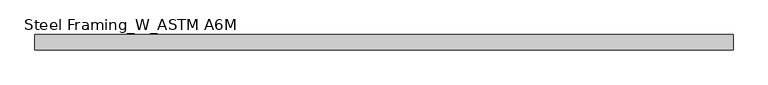
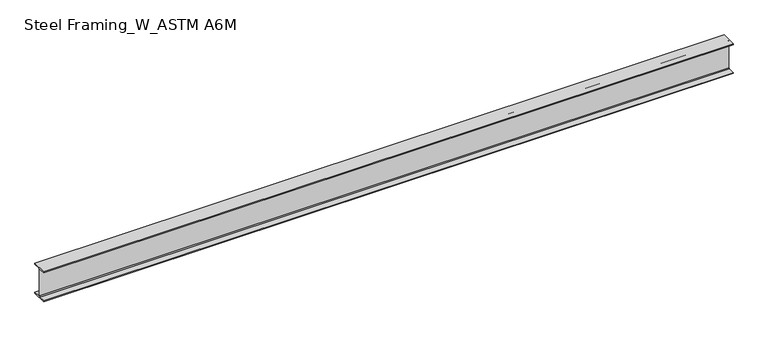
"""IFC4 building model written with IfcOpenShell, lengths in millimetres: beam geometry, Steel Framing_W_ASTM A6M : H_SB_AR_S02_W360x51_G3."""

import ifcopenshell
import ifcopenshell.guid

model = None  # the IFC model being written
_history = None  # IfcOwnerHistory: only IFC2X3 demands one
_inside = {}  # id of a spatial element -> (the spatial element, [elements in it])
_under = {}  # id of a project, library or spatial element -> (it, [spatial elements below it])
_declared = {}  # id of a project -> (the project, [libraries it declares])
_typed = {}  # id of a type object -> (the type object, [elements of that type])
_made_of = {}  # id of a material, layer set ... -> (it, [elements and type objects made of it])


def new_model(schema):
    """Start an empty IFC model of exactly this schema.

    Asked for "IFC4X3", IfcOpenShell would pick the latest addendum, in which some entities
    have other attributes; the version numbers below select the first issue.
    IFC2X3 requires an IfcOwnerHistory on every rooted entity: one is made here for all.
    """
    global model, _history
    if schema == "IFC4X3":
        model = ifcopenshell.file(schema_version=(4, 3, 0, 0))
    else:
        model = ifcopenshell.file(schema=schema)
    _inside.clear()
    _under.clear()
    _declared.clear()
    _typed.clear()
    _made_of.clear()
    _history = None
    if model.schema == "IFC2X3":
        org = make("IfcOrganization", Name="unknown")
        user = make(
            "IfcPersonAndOrganization",
            ThePerson=make("IfcPerson", FamilyName="unknown"),
            TheOrganization=org,
        )
        app = make(
            "IfcApplication",
            ApplicationDeveloper=org,
            Version="unknown",
            ApplicationFullName="unknown",
            ApplicationIdentifier="unknown",
        )
        _history = make(
            "IfcOwnerHistory",
            OwningUser=user,
            OwningApplication=app,
            ChangeAction="ADDED",
            CreationDate=0,
        )
    return model


def make(cls, **values):
    """One entity of the class cls with the attributes given. An attribute that is None is left unset."""
    return model.create_entity(
        cls, **{name: value for name, value in values.items() if value is not None}
    )


def rooted(cls, **values):
    """An entity with a GlobalId (a new one), such as an element, a storey or a relation."""
    return make(cls, GlobalId=ifcopenshell.guid.new(), OwnerHistory=_history, **values)


def si_unit(unit_type, name, prefix=None):
    """IfcSIUnit, for example si_unit("LENGTHUNIT", "METRE", prefix="MILLI")."""
    return make("IfcSIUnit", UnitType=unit_type, Prefix=prefix, Name=name)


def assignment(units):
    """IfcUnitAssignment: the units of a project."""
    return None if units is None else make("IfcUnitAssignment", Units=units)


def point(xyz):
    """IfcCartesianPoint."""
    return None if xyz is None else make("IfcCartesianPoint", Coordinates=xyz)


def direction(xyz):
    """IfcDirection."""
    return None if xyz is None else make("IfcDirection", DirectionRatios=xyz)


def frame(location, z_axis=None, x_axis=None):
    """IfcAxis2Placement3D, a coordinate frame: its origin and axes. An axis left out is left unset."""
    return make(
        "IfcAxis2Placement3D",
        Location=point(location),
        Axis=direction(z_axis),
        RefDirection=direction(x_axis),
    )


def frame_2d(location, x_axis=None):
    """IfcAxis2Placement2D, a coordinate frame in the plane: its origin and x axis."""
    return make(
        "IfcAxis2Placement2D", Location=point(location), RefDirection=direction(x_axis)
    )


def origin():
    """The frame at (0, 0, 0) with its axes left unset."""
    return frame((0.0, 0.0, 0.0))


def place(relative_to, where):
    """IfcLocalPlacement: puts the frame where relative to a parent placement (None: the world)."""
    return make(
        "IfcLocalPlacement", PlacementRelTo=relative_to, RelativePlacement=where
    )


def context(
    kind, dimensions, precision=None, world=None, true_north=None, identifier=None
):
    """IfcGeometricRepresentationContext, for example the 3D "Model" context."""
    return make(
        "IfcGeometricRepresentationContext",
        ContextIdentifier=identifier,
        ContextType=kind,
        CoordinateSpaceDimension=dimensions,
        Precision=precision,
        WorldCoordinateSystem=world,
        TrueNorth=true_north,
    )


def project(units=None, contexts=None):
    """IfcProject with its units and contexts."""
    return rooted(
        "IfcProject",
        Name="project",
        RepresentationContexts=contexts,
        UnitsInContext=assignment(units),
    )


def spatial(cls, under=None, at=None, **own):
    """A site, building, storey or space (cls), placed at a placement, below another one or the project."""
    s = rooted(cls, ObjectPlacement=at, **own)
    if under is not None:
        _under.setdefault(under.id(), (under, []))[1].append(s)
    return s


def polyline(points):
    """IfcPolyline through the points."""
    return make("IfcPolyline", Points=[point(p) for p in points])


def circle_curve(where, radius):
    """IfcCircle in the frame where."""
    return make("IfcCircle", Position=where, Radius=radius)


def trimmed(basis, trim1, trim2, sense, master):
    """IfcTrimmedCurve: the piece of a basis curve between two trims."""
    return make(
        "IfcTrimmedCurve",
        BasisCurve=basis,
        Trim1=trim1,
        Trim2=trim2,
        SenseAgreement=sense,
        MasterRepresentation=master,
    )


def segment(curve, same_sense, transition):
    """IfcCompositeCurveSegment."""
    return make(
        "IfcCompositeCurveSegment",
        Transition=transition,
        SameSense=same_sense,
        ParentCurve=curve,
    )


def composite_curve(segments, self_intersect=None):
    """IfcCompositeCurve: segments joined end to end."""
    return make("IfcCompositeCurve", Segments=segments, SelfIntersect=self_intersect)


def outline(outer, holes=None, kind="AREA"):
    """IfcArbitraryClosedProfileDef: a profile drawn as a closed curve; with holes, ...WithVoids."""
    if holes is None:
        return make("IfcArbitraryClosedProfileDef", ProfileType=kind, OuterCurve=outer)
    return make(
        "IfcArbitraryProfileDefWithVoids",
        ProfileType=kind,
        OuterCurve=outer,
        InnerCurves=holes,
    )


def extrude(swept, where, along, depth):
    """IfcExtrudedAreaSolid: the profile swept, set in the frame where, extruded along a direction by depth."""
    return make(
        "IfcExtrudedAreaSolid",
        SweptArea=swept,
        Position=where,
        ExtrudedDirection=direction(along),
        Depth=depth,
    )


def shape(context_of_items, identifier, shape_type, items):
    """IfcShapeRepresentation: the items that make up one representation, for example the "Body"."""
    return make(
        "IfcShapeRepresentation",
        ContextOfItems=context_of_items,
        RepresentationIdentifier=identifier,
        RepresentationType=shape_type,
        Items=items,
    )


def source(mapping_origin, context_of_items, identifier, shape_type, items):
    """IfcRepresentationMap: a shape defined once, which mapped items show again and again."""
    return make(
        "IfcRepresentationMap",
        MappingOrigin=mapping_origin,
        MappedRepresentation=shape(context_of_items, identifier, shape_type, items),
    )


def transform(
    local_origin,
    x_axis=None,
    y_axis=None,
    z_axis=None,
    scale=None,
    scale2=None,
    scale3=None,
    uniform=True,
):
    """IfcCartesianTransformationOperator3D, or its non-uniform kind. x_axis, y_axis, z_axis: its Axis1, 2, 3."""
    if uniform:
        return make(
            "IfcCartesianTransformationOperator3D",
            Axis1=direction(x_axis),
            Axis2=direction(y_axis),
            LocalOrigin=point(local_origin),
            Scale=scale,
            Axis3=direction(z_axis),
        )
    return make(
        "IfcCartesianTransformationOperator3DnonUniform",
        Axis1=direction(x_axis),
        Axis2=direction(y_axis),
        LocalOrigin=point(local_origin),
        Scale=scale,
        Axis3=direction(z_axis),
        Scale2=scale2,
        Scale3=scale3,
    )


def mapped(mapping_source, mapping_target):
    """IfcMappedItem: shows the shape of a source again, moved by a transform."""
    return make(
        "IfcMappedItem", MappingSource=mapping_source, MappingTarget=mapping_target
    )


def made_of(thing, what):
    """Note that an element or type object is made of a material, layer set ...; save() writes the relation."""
    if what is not None:
        _made_of.setdefault(what.id(), (what, []))[1].append(thing)
    return thing


def element(
    cls,
    number,
    at=None,
    inside=None,
    cuts=None,
    type_object=None,
    material=None,
    context=None,
    identifier="Body",
    shape_type=None,
    held_by="IfcProductDefinitionShape",
    body=None,
    shapes=None,
    **own,
):
    """One element of the class cls, such as IfcWall. Its Tag is "e" and its number.

    at: its placement. inside: the storey or other place that contains it. cuts: it is an
    opening in that element (IfcRelVoidsElement). A single representation is given by context,
    identifier, shape_type and body (its items); several are given by shapes. held_by: the class
    of the entity that holds the representations. save() writes the other relations.
    """
    e = rooted(cls, Tag="e%d" % number, ObjectPlacement=at, **own)
    if body is not None:
        shapes = [shape(context, identifier, shape_type, body)]
    if shapes is not None:
        e.Representation = make(held_by, Representations=shapes)
    if inside is not None:
        _inside.setdefault(inside.id(), (inside, []))[1].append(e)
    if cuts is not None:
        rooted(
            "IfcRelVoidsElement", RelatingBuildingElement=cuts, RelatedOpeningElement=e
        )
    if type_object is not None:
        _typed.setdefault(type_object.id(), (type_object, []))[1].append(e)
    return made_of(e, material)


def aggregate(whole, parts):
    """IfcRelAggregates: a whole, such as a stair, and the parts it consists of."""
    return rooted("IfcRelAggregates", RelatingObject=whole, RelatedObjects=parts)


def save(model, path):
    """Write the relations noted so far, then the file.

    IfcRelAggregates (storeys below a building ...), IfcRelContainedInSpatialStructure (elements
    in a storey), IfcRelDefinesByType, IfcRelAssociatesMaterial and IfcRelDeclares: one each for
    every whole, place, type object, material and project.
    """
    for whole, parts in _under.values():
        aggregate(whole, parts)
    for where, things in _inside.values():
        rooted(
            "IfcRelContainedInSpatialStructure",
            RelatedElements=things,
            RelatingStructure=where,
        )
    for kind, things in _typed.values():
        rooted("IfcRelDefinesByType", RelatedObjects=things, RelatingType=kind)
    for what, things in _made_of.values():
        rooted("IfcRelAssociatesMaterial", RelatedObjects=things, RelatingMaterial=what)
    for by, libraries in _declared.values():
        rooted("IfcRelDeclares", RelatingContext=by, RelatedDefinitions=libraries)
    model.write(path)


def steel_framing_w_astm_a6m_becc2698(model_context):
    return source(origin(), model_context, "Body", "SweptSolid", [
        extrude(outline(composite_curve([segment(polyline([(85.5, -166.4), (85.5, -178.0), (-85.5, -178.0), (-85.5, -166.4), (-13.72, -166.4)]), True, "CONTINUOUS"), segment(trimmed(circle_curve(frame_2d((-13.72, -156.3)), 10.1), [point((-13.72, -166.4))], [point((-3.62, -156.3))], True, "CARTESIAN"), True, "CONTINUOUS"), segment(polyline([(-3.62, -156.3), (-3.62, 156.3)]), True, "CONTINUOUS"), segment(trimmed(circle_curve(frame_2d((-13.72, 156.3)), 10.1), [point((-3.62, 156.3))], [point((-13.72, 166.4))], True, "CARTESIAN"), True, "CONTINUOUS"), segment(polyline([(-13.72, 166.4), (-85.5, 166.4), (-85.5, 178.0), (85.5, 178.0), (85.5, 166.4), (13.72, 166.4)]), True, "CONTINUOUS"), segment(trimmed(circle_curve(frame_2d((13.72, 156.3)), 10.1), [point((13.72, 166.4))], [point((3.62, 156.3))], True, "CARTESIAN"), True, "CONTINUOUS"), segment(polyline([(3.62, 156.3), (3.62, -156.3)]), True, "CONTINUOUS"), segment(trimmed(circle_curve(frame_2d((13.72, -156.3)), 10.1), [point((3.62, -156.3))], [point((13.72, -166.4))], True, "CARTESIAN"), True, "CONTINUOUS"), segment(polyline([(13.72, -166.4), (85.5, -166.4)]), True, "CONTINUOUS")], self_intersect=False)), frame((-3884.3, 0.0, 0.0), z_axis=(1.0, 0.0, 0.0), x_axis=(0.0, 1.0, 0.0)), (0.0, 0.0, 1.0), 7768.6),
    ])


if __name__ == "__main__":
    model = new_model("IFC4")
    model_context = context("Model", 3, world=origin())
    ifc_project = project(units=[si_unit("LENGTHUNIT", "METRE", prefix="MILLI")], contexts=[model_context])
    site = spatial("IfcSite", under=ifc_project)
    building = spatial("IfcBuilding", under=site)
    placement = place(None, origin())
    steel_framing_w_astm_a6m_shape = steel_framing_w_astm_a6m_becc2698(model_context)
    element("IfcBeam", 1, ObjectType="Steel Framing_W_ASTM A6M : H_SB_AR_S02_W360x51_G3", at=placement, inside=building, context=model_context, shape_type="MappedRepresentation", body=[
        mapped(steel_framing_w_astm_a6m_shape, transform((0.0, 0.0, 0.0), x_axis=(1.0, 0.0, 0.0), y_axis=(0.0, 1.0, 0.0), z_axis=(0.0, 0.0, 1.0))),
    ])
    save(model, "model.ifc")

# Revit data of these elements
# Type "Steel Framing_W_ASTM A6M : H_SB_AR_S02_W360x51_G3"
#   Type Mark = "G3"
#   Section Name Key = "W14x34"
#   Width = 17.1 cm
#   Web Thickness = 0.724 cm
#   Web Fillet = 1.01 cm
#   Warping Constant = 287000.0 cm⁶
#   Torsional Moment of Inertia = 23.70 cm⁴
#   Section Area = 64.5 cm²
#   Plastic Modulus weak axis = 174.0 cm³
#   Plastic Modulus strong axis = 895.0 cm³
#   Perimeter = 1.36 m²/m
#   Nominal Weight = 51.00 kgf/m
#   Moment of Inertia weak axis = 970.00 cm⁴
#   Moment of Inertia strong axis = 14200.00 cm⁴
#   Height = 35.6 cm
#   Flange Thickness = 1.16 cm
#   Elastic Modulus weak axis = 113.0 cm³
#   Elastic Modulus strong axis = 796.0 cm³
#   Centroid Vertical = 17.8 cm
#   Centroid Horizontal = 8.55 cm
#   Length [instance default] = 1500 mm
#   Structural Material [instance default] = Steel, 45-345
#   Bolt Spacing = 0
#   Assembly Code = ""
# Element 1 (IfcBeam, "Steel Framing_W_ASTM A6M : H_SB_AR_S02_W360x51_G3")
#   Materials on its faces: "Steel, 45-345"
# Materials
#   "Steel, 45-345": class "Metal", colour RGB 189 187 185, transparency 0, Description = "Steel 345 MPa", Cost = 0
